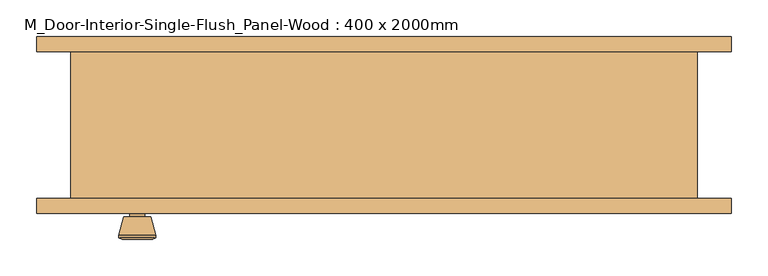
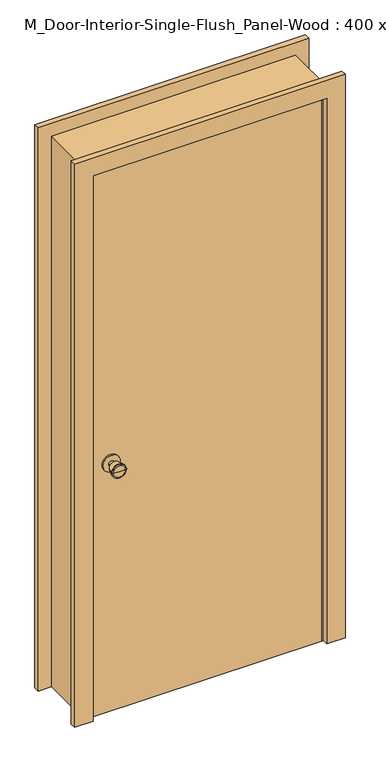
"""IFC4 building model written with IfcOpenShell, lengths in millimetres: door geometry, M_Door-Interior-Single-Flush_Panel-Wood : 400 x 2000mm."""

from ifc_helpers import new_model, si_unit, point, frame, frame_2d, origin, origin_with_axes, place, context, project, spatial, polyline, circle_curve, trimmed, segment, composite_curve, outline, extrude, faceted_brep, source, transform, mapped, element, save
from ifc_brep_helpers import plane_surface, cylinder_surface, revolved_surface, advanced_brep


def m_door_interior_single_flush_panel_wood_400_x_2000mm_2d1b6dcd(model_context):
    return source(origin(), model_context, "Body", "SolidModel", [
        advanced_brep(
        [(-335.0, -55.825, 914.4), (-345.0, -55.825, 914.4), (-325.0, -55.825, 914.4), (-314.5241324, -6.825, 914.4), (-355.4758676, -6.825, 914.4), (-335.0, -6.825, 914.4), (-310.0, -8.6528681, 914.4), (-360.0, -8.6528681, 914.4), (-310.0, -12.1165463, 914.4), (-360.0, -12.1165463, 914.4), (-316.363764, -36.825, 914.4), (-353.636236, -36.825, 914.4), (-325.0, -36.825, 914.4), (-345.0, -36.825, 914.4)],
        [
            (0, 1),
            (1, 2, circle_curve(frame((-335.0, -55.825, 914.4), z_axis=(0.0, -1.0, 0.0), x_axis=(-1.0, 0.0, 0.0)), 10.0)),
            (2, 0),
            (2, 1, circle_curve(frame((-335.0, -55.825, 914.4), z_axis=(0.0, -1.0, 0.0), x_axis=(-1.0, 0.0, 0.0)), 10.0)),
            (3, 4, circle_curve(frame((-335.0, -6.825, 914.4), z_axis=(0.0, 1.0, 0.0), x_axis=(-1.0, 0.0, 0.0)), 20.4758676)),
            (4, 5),
            (5, 3),
            (4, 3, circle_curve(frame((-335.0, -6.825, 914.4), z_axis=(0.0, 1.0, 0.0), x_axis=(-1.0, 0.0, 0.0)), 20.4758676)),
            (6, 7, circle_curve(frame((-335.0, -8.6528681, 914.4), z_axis=(0.0, 1.0, 0.0), x_axis=(-1.0, 0.0, 0.0)), 25.0)),
            (7, 4),
            (3, 6),
            (7, 6, circle_curve(frame((-335.0, -8.6528681, 914.4), z_axis=(0.0, 1.0, 0.0), x_axis=(-1.0, 0.0, 0.0)), 25.0)),
            (8, 9, circle_curve(frame((-335.0, -12.1165463, 914.4), z_axis=(0.0, 1.0, 0.0), x_axis=(-1.0, 0.0, 0.0)), 25.0)),
            (9, 7),
            (6, 8),
            (9, 8, circle_curve(frame((-335.0, -12.1165463, 914.4), z_axis=(0.0, 1.0, 0.0), x_axis=(-1.0, 0.0, 0.0)), 25.0)),
            (10, 11, circle_curve(frame((-335.0, -36.825, 914.4), z_axis=(0.0, 1.0, 0.0), x_axis=(-1.0, 0.0, 0.0)), 18.636236)),
            (11, 9),
            (8, 10),
            (11, 10, circle_curve(frame((-335.0, -36.825, 914.4), z_axis=(0.0, 1.0, 0.0), x_axis=(-1.0, 0.0, 0.0)), 18.636236)),
            (12, 13, circle_curve(frame((-335.0, -36.825, 914.4), z_axis=(0.0, 1.0, 0.0), x_axis=(-1.0, 0.0, 0.0)), 10.0)),
            (13, 11),
            (10, 12),
            (13, 12, circle_curve(frame((-335.0, -36.825, 914.4), z_axis=(0.0, 1.0, 0.0), x_axis=(-1.0, 0.0, 0.0)), 10.0)),
            (1, 13),
            (12, 2),
        ],
        [
            plane_surface(frame((-335.0, -55.825, 914.4), z_axis=(0.0, -1.0, 0.0), x_axis=(-1.0, 0.0, 0.0))),
            plane_surface(frame((-335.0, -6.825, 914.4), z_axis=(0.0, 1.0, 0.0), x_axis=(-1.0, 0.0, 0.0))),
            revolved_surface(polyline([(-355.4758676, -6.825, 914.4), (-360.0, -8.6528681, 914.4)]), (-335.0, -55.825, 914.4), (0.0, -1.0, 0.0)),
            cylinder_surface(frame((-335.0, -55.825, 914.4), z_axis=(0.0, -1.0, 0.0), x_axis=(-1.0, 0.0, 0.0)), 25.0),
            revolved_surface(polyline([(-360.0, -12.1165463, 914.4), (-353.636236, -36.825, 914.4)]), (-335.0, -55.825, 914.4), (0.0, -1.0, 0.0)),
            plane_surface(frame((-335.0, -36.825, 914.4), z_axis=(0.0, -1.0, 0.0), x_axis=(-1.0, 0.0, 0.0))),
            cylinder_surface(frame((-335.0, -55.825, 914.4), z_axis=(0.0, -1.0, 0.0), x_axis=(-1.0, 0.0, 0.0)), 10.0),
        ],
        [
            (0, [[1, 2, 3]]),
            (0, [[-3, 4, -1]]),
            (1, [[5, 6, 7]]),
            (1, [[8, -7, -6]]),
            (2, [[9, 10, -5, 11]]),
            (2, [[12, -11, -8, -10]]),
            (3, [[13, 14, -9, 15]]),
            (3, [[16, -15, -12, -14]]),
            (4, [[17, 18, -13, 19]]),
            (4, [[20, -19, -16, -18]]),
            (5, [[21, 22, -17, 23]]),
            (5, [[24, -23, -20, -22]]),
            (6, [[-2, 25, -21, 26]]),
            (6, [[-4, -26, -24, -25]]),
        ],
    ),
        extrude(outline(composite_curve([segment(trimmed(circle_curve(frame_2d((914.4, -335.0)), 30.0), [point((914.4, -365.0))], [point((914.4, -305.0))], False, "CARTESIAN"), True, "CONTINUOUS"), segment(trimmed(circle_curve(frame_2d((914.4, -335.0)), 30.0), [point((914.4, -305.0))], [point((914.4, -365.0))], False, "CARTESIAN"), True, "CONTINUOUS")], self_intersect=False)), frame((0.0, -61.825, 0.0), z_axis=(0.0, 1.0, 0.0), x_axis=(0.0, 0.0, 1.0)), (0.0, 0.0, 1.0), 6.0),
        advanced_brep(
        [(-335.0, -102.825, 914.4), (-325.0, -102.825, 914.4), (-345.0, -102.825, 914.4), (-314.5241324, -151.825, 914.4), (-335.0, -151.825, 914.4), (-355.4758676, -151.825, 914.4), (-310.0, -149.9971319, 914.4), (-360.0, -149.9971319, 914.4), (-310.0, -146.5334537, 914.4), (-360.0, -146.5334537, 914.4), (-316.363764, -121.825, 914.4), (-353.636236, -121.825, 914.4), (-325.0, -121.825, 914.4), (-345.0, -121.825, 914.4)],
        [
            (0, 1),
            (1, 2, circle_curve(frame((-335.0, -102.825, 914.4), z_axis=(0.0, 1.0, 0.0), x_axis=(-1.0, 0.0, 0.0)), 10.0)),
            (2, 0),
            (2, 1, circle_curve(frame((-335.0, -102.825, 914.4), z_axis=(0.0, 1.0, 0.0), x_axis=(-1.0, 0.0, 0.0)), 10.0)),
            (3, 4),
            (4, 5),
            (5, 3, circle_curve(frame((-335.0, -151.825, 914.4), z_axis=(0.0, -1.0, 0.0), x_axis=(-1.0, 0.0, 0.0)), 20.4758676)),
            (3, 5, circle_curve(frame((-335.0, -151.825, 914.4), z_axis=(0.0, -1.0, 0.0), x_axis=(-1.0, 0.0, 0.0)), 20.4758676)),
            (6, 3),
            (5, 7),
            (7, 6, circle_curve(frame((-335.0, -149.9971319, 914.4), z_axis=(0.0, -1.0, 0.0), x_axis=(-1.0, 0.0, 0.0)), 25.0)),
            (6, 7, circle_curve(frame((-335.0, -149.9971319, 914.4), z_axis=(0.0, -1.0, 0.0), x_axis=(-1.0, 0.0, 0.0)), 25.0)),
            (8, 6),
            (7, 9),
            (9, 8, circle_curve(frame((-335.0, -146.5334537, 914.4), z_axis=(0.0, -1.0, 0.0), x_axis=(-1.0, 0.0, 0.0)), 25.0)),
            (8, 9, circle_curve(frame((-335.0, -146.5334537, 914.4), z_axis=(0.0, -1.0, 0.0), x_axis=(-1.0, 0.0, 0.0)), 25.0)),
            (10, 8),
            (9, 11),
            (11, 10, circle_curve(frame((-335.0, -121.825, 914.4), z_axis=(0.0, -1.0, 0.0), x_axis=(-1.0, 0.0, 0.0)), 18.636236)),
            (10, 11, circle_curve(frame((-335.0, -121.825, 914.4), z_axis=(0.0, -1.0, 0.0), x_axis=(-1.0, 0.0, 0.0)), 18.636236)),
            (12, 10),
            (11, 13),
            (13, 12, circle_curve(frame((-335.0, -121.825, 914.4), z_axis=(0.0, -1.0, 0.0), x_axis=(-1.0, 0.0, 0.0)), 10.0)),
            (12, 13, circle_curve(frame((-335.0, -121.825, 914.4), z_axis=(0.0, -1.0, 0.0), x_axis=(-1.0, 0.0, 0.0)), 10.0)),
            (1, 12),
            (13, 2),
        ],
        [
            plane_surface(frame((-335.0, -102.825, 914.4), z_axis=(0.0, 1.0, 0.0), x_axis=(-1.0, 0.0, 0.0))),
            plane_surface(frame((-335.0, -151.825, 914.4), z_axis=(0.0, -1.0, 0.0), x_axis=(-1.0, 0.0, 0.0))),
            revolved_surface(polyline([(-355.4758676, -151.825, 914.4), (-360.0, -149.9971319, 914.4)]), (-335.0, -102.825, 914.4), (0.0, 1.0, 0.0)),
            cylinder_surface(frame((-335.0, -102.825, 914.4), z_axis=(0.0, 1.0, 0.0), x_axis=(-1.0, 0.0, 0.0)), 25.0),
            revolved_surface(polyline([(-360.0, -146.5334537, 914.4), (-353.636236, -121.825, 914.4)]), (-335.0, -102.825, 914.4), (0.0, 1.0, 0.0)),
            plane_surface(frame((-335.0, -121.825, 914.4), z_axis=(0.0, 1.0, 0.0), x_axis=(-1.0, 0.0, 0.0))),
            cylinder_surface(frame((-335.0, -102.825, 914.4), z_axis=(0.0, 1.0, 0.0), x_axis=(-1.0, 0.0, 0.0)), 10.0),
        ],
        [
            (0, [[1, 2, 3]]),
            (0, [[-3, 4, -1]]),
            (1, [[5, 6, 7]]),
            (1, [[-6, -5, 8]]),
            (2, [[9, -7, 10, 11]]),
            (2, [[-10, -8, -9, 12]]),
            (3, [[13, -11, 14, 15]]),
            (3, [[-14, -12, -13, 16]]),
            (4, [[17, -15, 18, 19]]),
            (4, [[-18, -16, -17, 20]]),
            (5, [[21, -19, 22, 23]]),
            (5, [[-22, -20, -21, 24]]),
            (6, [[25, -23, 26, -2]]),
            (6, [[-26, -24, -25, -4]]),
        ],
    ),
        extrude(outline(composite_curve([segment(trimmed(circle_curve(frame_2d((914.4, -335.0)), 30.0), [point((914.4, -365.0))], [point((914.4, -305.0))], False, "CARTESIAN"), True, "CONTINUOUS"), segment(trimmed(circle_curve(frame_2d((914.4, -335.0)), 30.0), [point((914.4, -305.0))], [point((914.4, -365.0))], False, "CARTESIAN"), True, "CONTINUOUS")], self_intersect=False)), frame((0.0, -102.825, 0.0), z_axis=(0.0, 1.0, 0.0), x_axis=(0.0, 0.0, 1.0)), (0.0, 0.0, 1.0), 6.0),
        extrude(outline(polyline([(400.0, -61.825), (400.0, -96.825), (-400.0, -96.825), (-400.0, -61.825), (400.0, -61.825)])), origin_with_axes(), (0.0, 0.0, 1.0), 2000.0),
        faceted_brep([(425.0, -96.825, 0.0), (400.0, -96.825, 0.0), (400.0, -61.825, 0.0), (387.3, -61.825, 0.0), (387.3, -26.9, 0.0), (400.0, -26.9, 0.0), (400.0, 103.175, 0.0), (425.0, 103.175, 0.0), (425.0, 103.175, 2025.0), (425.0, -96.825, 2025.0), (400.0, 103.175, 2000.0), (-400.0, 103.175, 2000.0), (-400.0, 103.175, 0.0), (-425.0, 103.175, 0.0), (-425.0, 103.175, 2025.0), (400.0, -26.9, 2000.0), (387.3, -26.9, 1987.3), (-387.3, -26.9, 1987.3), (-387.3, -26.9, 0.0), (-400.0, -26.9, 0.0), (-400.0, -26.9, 2000.0), (387.3, -61.825, 1987.3), (400.0, -61.825, 2000.0), (-400.0, -61.825, 2000.0), (-400.0, -61.825, 0.0), (-387.3, -61.825, 0.0), (-387.3, -61.825, 1987.3), (400.0, -96.825, 2000.0), (-425.0, -96.825, 2025.0), (-425.0, -96.825, 0.0), (-400.0, -96.825, 0.0), (-400.0, -96.825, 2000.0)], [[[0, 1, 2, 3, 4, 5, 6, 7]], [[7, 8, 9, 0]], [[6, 10, 11, 12, 13, 14, 8, 7]], [[5, 15, 10, 6]], [[4, 16, 17, 18, 19, 20, 15, 5]], [[3, 21, 16, 4]], [[2, 22, 23, 24, 25, 26, 21, 3]], [[1, 27, 22, 2]], [[0, 9, 28, 29, 30, 31, 27, 1]], [[8, 14, 28, 9]], [[15, 20, 11, 10]], [[21, 26, 17, 16]], [[27, 31, 23, 22]], [[29, 13, 12, 19, 18, 25, 24, 30]], [[14, 13, 29, 28]], [[20, 19, 12, 11]], [[26, 25, 18, 17]], [[31, 30, 24, 23]]]),
        extrude(outline(polyline([(0.0, 471.35), (2071.35, 471.35), (2071.35, -471.35), (0.0, -471.35), (0.0, -406.35), (2006.35, -406.35), (2006.35, 406.35), (0.0, 406.35), (0.0, 471.35)])), frame((0.0, 103.175, 0.0), z_axis=(0.0, 1.0, 0.0), x_axis=(0.0, 0.0, 1.0)), (0.0, 0.0, 1.0), 20.0),
        extrude(outline(polyline([(0.0, 471.35), (2071.35, 471.35), (2071.35, -471.35), (0.0, -471.35), (0.0, -406.35), (2006.35, -406.35), (2006.35, 406.35), (0.0, 406.35), (0.0, 471.35)])), frame((0.0, -116.825, 0.0), z_axis=(0.0, 1.0, 0.0), x_axis=(0.0, 0.0, 1.0)), (0.0, 0.0, 1.0), 20.0),
    ])


if __name__ == "__main__":
    model = new_model("IFC4")
    model_context = context("Model", 3, world=origin())
    ifc_project = project(units=[si_unit("LENGTHUNIT", "METRE", prefix="MILLI")], contexts=[model_context])
    site = spatial("IfcSite", under=ifc_project)
    building = spatial("IfcBuilding", under=site)
    placement = place(None, origin())
    m_door_interior_single_flush_panel_wood_400_x_2000mm_shape = m_door_interior_single_flush_panel_wood_400_x_2000mm_2d1b6dcd(model_context)
    element("IfcDoor", 1, ObjectType="M_Door-Interior-Single-Flush_Panel-Wood : 400 x 2000mm", at=placement, inside=building, context=model_context, shape_type="MappedRepresentation", body=[
        mapped(m_door_interior_single_flush_panel_wood_400_x_2000mm_shape, transform((0.0, 0.0, 0.0), x_axis=(1.0, 0.0, 0.0), y_axis=(0.0, 1.0, 0.0), z_axis=(0.0, 0.0, 1.0))),
    ])
    save(model, "model.ifc")

# Revit data of these elements
# Type "M_Door-Interior-Single-Flush_Panel-Wood : 400 x 2000mm"
#   Type Mark = "22"
#   Assembly Code = "C1020300"
#   Analytic Construction = "Wooden"
#   Thickness = 0.035 m
#   Thermal Resistance (R) = 0.455703 (m²·K)/W
#   Swing Angle [instance default] = 90.00°
#   Rough Width = 0.85 m
#   Rough Height = 2.025 m
#   Height = 2 m
#   Width = 0.8 m
#   Heat Transfer Coefficient (U) = 2.19465 W/(m²·K)
#   Trim Material = Cherry
#   Panel Material = Cherry
#   Frame Material = Cherry
#   Door Handle Material = Aluminum
#   Visual Light Transmittance = 0
#   Solar Heat Gain Coefficient = 0
#   Wall Closure = (empty or 0)
#   Function = (empty or 0)
# Element 1 (IfcDoor, "M_Door-Interior-Single-Flush_Panel-Wood : 400 x 2000mm")
#   Materials on its faces: "Cherry", "Aluminum"
# Materials
#   "Cherry": class "Wood", colour RGB 226 177 128, transparency 0, Description = "Prunus Serotina", Cost = 0
#   "Aluminum": class "Metal", colour RGB 247 247 247, transparency 0, Description = "Aluminum 6061", Cost = 0
